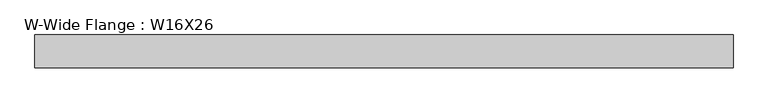
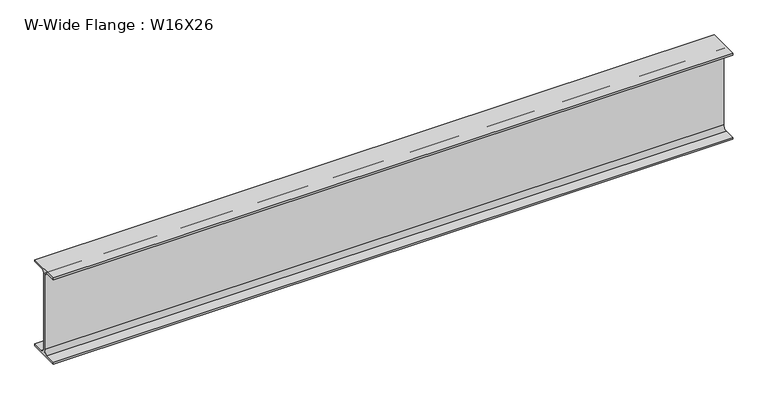
"""IFC4 building model written with IfcOpenShell, lengths in millimetres: beam geometry, W-Wide Flange : W16X26."""

from ifc_helpers import new_model, si_unit, point, frame, frame_2d, origin, place, context, project, spatial, polyline, circle_curve, trimmed, segment, composite_curve, outline, extrude, source, transform, mapped, element, save


def w_wide_flange_w16x26_f8cfc884(model_context):
    return source(origin(), model_context, "Body", "SweptSolid", [
        extrude(outline(composite_curve([segment(polyline([(69.85, -190.627), (69.85, -199.39), (-69.85, -199.39), (-69.85, -190.627), (-21.3995, -190.627)]), True, "CONTINUOUS"), segment(trimmed(circle_curve(frame_2d((-21.3995, -172.4025)), 18.2245), [point((-21.3995, -190.627))], [point((-3.175, -172.4025))], True, "CARTESIAN"), True, "CONTINUOUS"), segment(polyline([(-3.175, -172.4025), (-3.175, 172.4025)]), True, "CONTINUOUS"), segment(trimmed(circle_curve(frame_2d((-21.3995, 172.4025)), 18.2245), [point((-3.175, 172.4025))], [point((-21.3995, 190.627))], True, "CARTESIAN"), True, "CONTINUOUS"), segment(polyline([(-21.3995, 190.627), (-69.85, 190.627), (-69.85, 199.39), (69.85, 199.39), (69.85, 190.627), (21.3995, 190.627)]), True, "CONTINUOUS"), segment(trimmed(circle_curve(frame_2d((21.3995, 172.4025)), 18.2245), [point((21.3995, 190.627))], [point((3.175, 172.4025))], True, "CARTESIAN"), True, "CONTINUOUS"), segment(polyline([(3.175, 172.4025), (3.175, -172.4025)]), True, "CONTINUOUS"), segment(trimmed(circle_curve(frame_2d((21.3995, -172.4025)), 18.2245), [point((3.175, -172.4025))], [point((21.3995, -190.627))], True, "CARTESIAN"), True, "CONTINUOUS"), segment(polyline([(21.3995, -190.627), (69.85, -190.627)]), True, "CONTINUOUS")], self_intersect=False)), frame((-1475.1503394, 0.0, 0.0), z_axis=(1.0, 0.0, 0.0), x_axis=(0.0, 1.0, 0.0)), (0.0, 0.0, 1.0), 2973.2296556),
    ])


if __name__ == "__main__":
    model = new_model("IFC4")
    model_context = context("Model", 3, world=origin())
    ifc_project = project(units=[si_unit("LENGTHUNIT", "METRE", prefix="MILLI")], contexts=[model_context])
    site = spatial("IfcSite", under=ifc_project)
    building = spatial("IfcBuilding", under=site)
    placement = place(None, origin())
    w_wide_flange_w16x26_shape = w_wide_flange_w16x26_f8cfc884(model_context)
    element("IfcBeam", 1, ObjectType="W-Wide Flange : W16X26", at=placement, inside=building, context=model_context, shape_type="MappedRepresentation", body=[
        mapped(w_wide_flange_w16x26_shape, transform((0.0, 0.0, 0.0), x_axis=(1.0, 0.0, 0.0), y_axis=(0.0, 1.0, 0.0), z_axis=(0.0, 0.0, 1.0))),
    ])
    save(model, "model.ifc")

# Revit data of these elements
# Type "W-Wide Flange : W16X26"
#   Assembly Code = "B10"
#   W = 26
#   Length [instance default] = 5' - 0"
#   bf = 0' - 5 1/2"
#   d = 1' - 3.7"
#   k = 0' - 1 1/16"
#   k2 = 0' - 0.7175"
#   tf = 0' - 0.345"
#   tw = 0' - 0 1/4"
#   A = 0.0533333 SF
#   Structural Material [instance default] = Steel ASTM A992
# Element 1 (IfcBeam, "W-Wide Flange : W16X26")
#   Structural Material = Steel ASTM A36
#   Materials on its faces: "Steel ASTM A36"
# Materials
#   "Steel ASTM A992": class "Metal", colour RGB 199 199 199, transparency 0, Description = "Structural steel 50ksi", Cost = 0
#   "Steel ASTM A36": class "Metal", colour RGB 199 199 199, transparency 0, Description = "Structural steel, ASTM A36 Grade B, mill finish", Cost = 0
